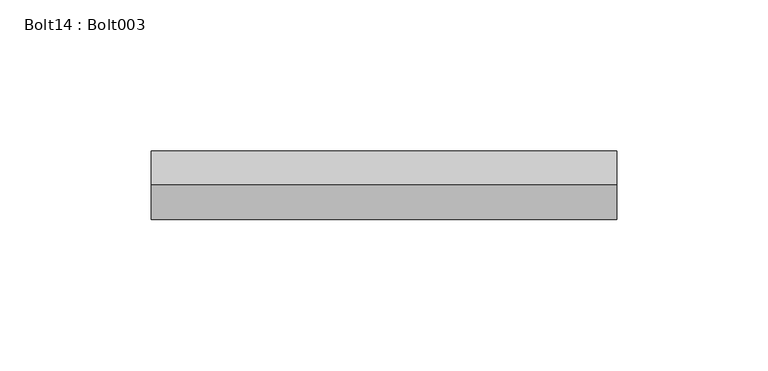
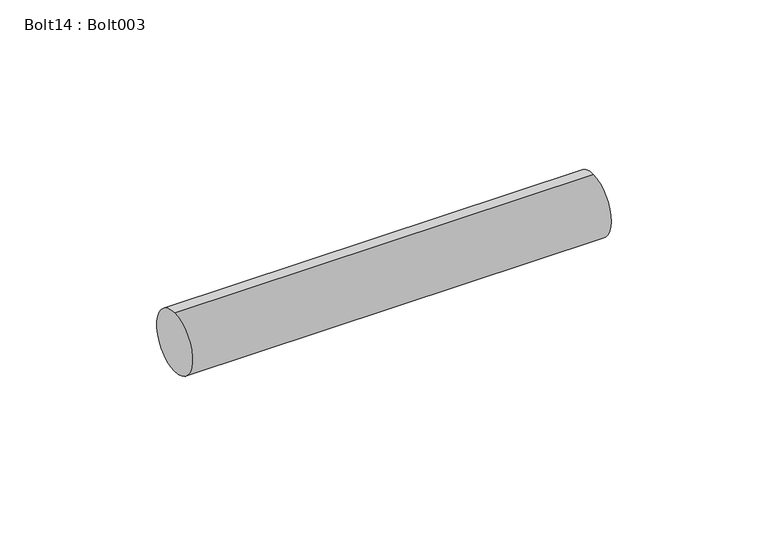
"""IFC4 building model written with IfcOpenShell, lengths in millimetres: proxy geometry, Bolt14 : Bolt003."""

import ifcopenshell
import ifcopenshell.guid

model = None  # the IFC model being written
_history = None  # IfcOwnerHistory: only IFC2X3 demands one
_inside = {}  # id of a spatial element -> (the spatial element, [elements in it])
_under = {}  # id of a project, library or spatial element -> (it, [spatial elements below it])
_declared = {}  # id of a project -> (the project, [libraries it declares])
_typed = {}  # id of a type object -> (the type object, [elements of that type])
_made_of = {}  # id of a material, layer set ... -> (it, [elements and type objects made of it])


def new_model(schema):
    """Start an empty IFC model of exactly this schema.

    Asked for "IFC4X3", IfcOpenShell would pick the latest addendum, in which some entities
    have other attributes; the version numbers below select the first issue.
    IFC2X3 requires an IfcOwnerHistory on every rooted entity: one is made here for all.
    """
    global model, _history
    if schema == "IFC4X3":
        model = ifcopenshell.file(schema_version=(4, 3, 0, 0))
    else:
        model = ifcopenshell.file(schema=schema)
    _inside.clear()
    _under.clear()
    _declared.clear()
    _typed.clear()
    _made_of.clear()
    _history = None
    if model.schema == "IFC2X3":
        org = make("IfcOrganization", Name="unknown")
        user = make(
            "IfcPersonAndOrganization",
            ThePerson=make("IfcPerson", FamilyName="unknown"),
            TheOrganization=org,
        )
        app = make(
            "IfcApplication",
            ApplicationDeveloper=org,
            Version="unknown",
            ApplicationFullName="unknown",
            ApplicationIdentifier="unknown",
        )
        _history = make(
            "IfcOwnerHistory",
            OwningUser=user,
            OwningApplication=app,
            ChangeAction="ADDED",
            CreationDate=0,
        )
    return model


def make(cls, **values):
    """One entity of the class cls with the attributes given. An attribute that is None is left unset."""
    return model.create_entity(
        cls, **{name: value for name, value in values.items() if value is not None}
    )


def rooted(cls, **values):
    """An entity with a GlobalId (a new one), such as an element, a storey or a relation."""
    return make(cls, GlobalId=ifcopenshell.guid.new(), OwnerHistory=_history, **values)


def si_unit(unit_type, name, prefix=None):
    """IfcSIUnit, for example si_unit("LENGTHUNIT", "METRE", prefix="MILLI")."""
    return make("IfcSIUnit", UnitType=unit_type, Prefix=prefix, Name=name)


def assignment(units):
    """IfcUnitAssignment: the units of a project."""
    return None if units is None else make("IfcUnitAssignment", Units=units)


def point(xyz):
    """IfcCartesianPoint."""
    return None if xyz is None else make("IfcCartesianPoint", Coordinates=xyz)


def direction(xyz):
    """IfcDirection."""
    return None if xyz is None else make("IfcDirection", DirectionRatios=xyz)


def frame(location, z_axis=None, x_axis=None):
    """IfcAxis2Placement3D, a coordinate frame: its origin and axes. An axis left out is left unset."""
    return make(
        "IfcAxis2Placement3D",
        Location=point(location),
        Axis=direction(z_axis),
        RefDirection=direction(x_axis),
    )


def frame_2d(location, x_axis=None):
    """IfcAxis2Placement2D, a coordinate frame in the plane: its origin and x axis."""
    return make(
        "IfcAxis2Placement2D", Location=point(location), RefDirection=direction(x_axis)
    )


def origin():
    """The frame at (0, 0, 0) with its axes left unset."""
    return frame((0.0, 0.0, 0.0))


def place(relative_to, where):
    """IfcLocalPlacement: puts the frame where relative to a parent placement (None: the world)."""
    return make(
        "IfcLocalPlacement", PlacementRelTo=relative_to, RelativePlacement=where
    )


def context(
    kind, dimensions, precision=None, world=None, true_north=None, identifier=None
):
    """IfcGeometricRepresentationContext, for example the 3D "Model" context."""
    return make(
        "IfcGeometricRepresentationContext",
        ContextIdentifier=identifier,
        ContextType=kind,
        CoordinateSpaceDimension=dimensions,
        Precision=precision,
        WorldCoordinateSystem=world,
        TrueNorth=true_north,
    )


def project(units=None, contexts=None):
    """IfcProject with its units and contexts."""
    return rooted(
        "IfcProject",
        Name="project",
        RepresentationContexts=contexts,
        UnitsInContext=assignment(units),
    )


def spatial(cls, under=None, at=None, **own):
    """A site, building, storey or space (cls), placed at a placement, below another one or the project."""
    s = rooted(cls, ObjectPlacement=at, **own)
    if under is not None:
        _under.setdefault(under.id(), (under, []))[1].append(s)
    return s


def circle_curve(where, radius):
    """IfcCircle in the frame where."""
    return make("IfcCircle", Position=where, Radius=radius)


def trimmed(basis, trim1, trim2, sense, master):
    """IfcTrimmedCurve: the piece of a basis curve between two trims."""
    return make(
        "IfcTrimmedCurve",
        BasisCurve=basis,
        Trim1=trim1,
        Trim2=trim2,
        SenseAgreement=sense,
        MasterRepresentation=master,
    )


def segment(curve, same_sense, transition):
    """IfcCompositeCurveSegment."""
    return make(
        "IfcCompositeCurveSegment",
        Transition=transition,
        SameSense=same_sense,
        ParentCurve=curve,
    )


def composite_curve(segments, self_intersect=None):
    """IfcCompositeCurve: segments joined end to end."""
    return make("IfcCompositeCurve", Segments=segments, SelfIntersect=self_intersect)


def outline(outer, holes=None, kind="AREA"):
    """IfcArbitraryClosedProfileDef: a profile drawn as a closed curve; with holes, ...WithVoids."""
    if holes is None:
        return make("IfcArbitraryClosedProfileDef", ProfileType=kind, OuterCurve=outer)
    return make(
        "IfcArbitraryProfileDefWithVoids",
        ProfileType=kind,
        OuterCurve=outer,
        InnerCurves=holes,
    )


def extrude(swept, where, along, depth):
    """IfcExtrudedAreaSolid: the profile swept, set in the frame where, extruded along a direction by depth."""
    return make(
        "IfcExtrudedAreaSolid",
        SweptArea=swept,
        Position=where,
        ExtrudedDirection=direction(along),
        Depth=depth,
    )


def shape(context_of_items, identifier, shape_type, items):
    """IfcShapeRepresentation: the items that make up one representation, for example the "Body"."""
    return make(
        "IfcShapeRepresentation",
        ContextOfItems=context_of_items,
        RepresentationIdentifier=identifier,
        RepresentationType=shape_type,
        Items=items,
    )


def source(mapping_origin, context_of_items, identifier, shape_type, items):
    """IfcRepresentationMap: a shape defined once, which mapped items show again and again."""
    return make(
        "IfcRepresentationMap",
        MappingOrigin=mapping_origin,
        MappedRepresentation=shape(context_of_items, identifier, shape_type, items),
    )


def transform(
    local_origin,
    x_axis=None,
    y_axis=None,
    z_axis=None,
    scale=None,
    scale2=None,
    scale3=None,
    uniform=True,
):
    """IfcCartesianTransformationOperator3D, or its non-uniform kind. x_axis, y_axis, z_axis: its Axis1, 2, 3."""
    if uniform:
        return make(
            "IfcCartesianTransformationOperator3D",
            Axis1=direction(x_axis),
            Axis2=direction(y_axis),
            LocalOrigin=point(local_origin),
            Scale=scale,
            Axis3=direction(z_axis),
        )
    return make(
        "IfcCartesianTransformationOperator3DnonUniform",
        Axis1=direction(x_axis),
        Axis2=direction(y_axis),
        LocalOrigin=point(local_origin),
        Scale=scale,
        Axis3=direction(z_axis),
        Scale2=scale2,
        Scale3=scale3,
    )


def mapped(mapping_source, mapping_target):
    """IfcMappedItem: shows the shape of a source again, moved by a transform."""
    return make(
        "IfcMappedItem", MappingSource=mapping_source, MappingTarget=mapping_target
    )


def made_of(thing, what):
    """Note that an element or type object is made of a material, layer set ...; save() writes the relation."""
    if what is not None:
        _made_of.setdefault(what.id(), (what, []))[1].append(thing)
    return thing


def element(
    cls,
    number,
    at=None,
    inside=None,
    cuts=None,
    type_object=None,
    material=None,
    context=None,
    identifier="Body",
    shape_type=None,
    held_by="IfcProductDefinitionShape",
    body=None,
    shapes=None,
    **own,
):
    """One element of the class cls, such as IfcWall. Its Tag is "e" and its number.

    at: its placement. inside: the storey or other place that contains it. cuts: it is an
    opening in that element (IfcRelVoidsElement). A single representation is given by context,
    identifier, shape_type and body (its items); several are given by shapes. held_by: the class
    of the entity that holds the representations. save() writes the other relations.
    """
    e = rooted(cls, Tag="e%d" % number, ObjectPlacement=at, **own)
    if body is not None:
        shapes = [shape(context, identifier, shape_type, body)]
    if shapes is not None:
        e.Representation = make(held_by, Representations=shapes)
    if inside is not None:
        _inside.setdefault(inside.id(), (inside, []))[1].append(e)
    if cuts is not None:
        rooted(
            "IfcRelVoidsElement", RelatingBuildingElement=cuts, RelatedOpeningElement=e
        )
    if type_object is not None:
        _typed.setdefault(type_object.id(), (type_object, []))[1].append(e)
    return made_of(e, material)


def aggregate(whole, parts):
    """IfcRelAggregates: a whole, such as a stair, and the parts it consists of."""
    return rooted("IfcRelAggregates", RelatingObject=whole, RelatedObjects=parts)


def save(model, path):
    """Write the relations noted so far, then the file.

    IfcRelAggregates (storeys below a building ...), IfcRelContainedInSpatialStructure (elements
    in a storey), IfcRelDefinesByType, IfcRelAssociatesMaterial and IfcRelDeclares: one each for
    every whole, place, type object, material and project.
    """
    for whole, parts in _under.values():
        aggregate(whole, parts)
    for where, things in _inside.values():
        rooted(
            "IfcRelContainedInSpatialStructure",
            RelatedElements=things,
            RelatingStructure=where,
        )
    for kind, things in _typed.values():
        rooted("IfcRelDefinesByType", RelatedObjects=things, RelatingType=kind)
    for what, things in _made_of.values():
        rooted("IfcRelAssociatesMaterial", RelatedObjects=things, RelatingMaterial=what)
    for by, libraries in _declared.values():
        rooted("IfcRelDeclares", RelatingContext=by, RelatedDefinitions=libraries)
    model.write(path)


def bolt14_bolt003_cd8d5e77(model_context):
    return source(origin(), model_context, "Body", "SweptSolid", [
        extrude(outline(composite_curve([segment(trimmed(circle_curve(frame_2d((1896.5882072, 40070.0545241)), 11.4045168), [point((1896.5882072, 40058.6500073))], [point((1896.5882072, 40081.4590409))], False, "CARTESIAN"), True, "CONTINUOUS"), segment(trimmed(circle_curve(frame_2d((1896.5882072, 40070.0545241)), 11.4045168), [point((1896.5882072, 40081.4590409))], [point((1896.5882072, 40058.6500073))], False, "CARTESIAN"), True, "CONTINUOUS")], self_intersect=False)), frame((10287.3140827, 0.0, 0.0), z_axis=(1.0, 0.0, 0.0), x_axis=(0.0, 1.0, 0.0)), (0.0, 0.0, 1.0), 154.0602393),
    ])


if __name__ == "__main__":
    model = new_model("IFC4")
    model_context = context("Model", 3, world=origin())
    ifc_project = project(units=[si_unit("LENGTHUNIT", "METRE", prefix="MILLI")], contexts=[model_context])
    site = spatial("IfcSite", under=ifc_project)
    building = spatial("IfcBuilding", under=site)
    placement = place(None, origin())
    bolt14_bolt003_shape = bolt14_bolt003_cd8d5e77(model_context)
    element("IfcBuildingElementProxy", 1, Name="Bolt14 : Bolt003", ObjectType="Bolt14 : Bolt003", at=placement, inside=building, context=model_context, shape_type="MappedRepresentation", body=[
        mapped(bolt14_bolt003_shape, transform((0.0, 0.0, 0.0), x_axis=(1.0, 0.0, 0.0), y_axis=(0.0, 1.0, 0.0), z_axis=(0.0, 0.0, 1.0))),
    ])
    save(model, "model.ifc")

# Revit data of these elements
# Type "Bolt14 : Bolt003"
#   NameOverride = "Bolt003"
# Element 1 (IfcBuildingElementProxy, "Bolt14 : Bolt003")
#   Materials on its faces: "TUBE STEEL STRINGER WELDED TO ANCHORED STEEL PLATE - SEE STRUCT DWGS"
# Materials
#   "TUBE STEEL STRINGER WELDED TO ANCHORED STEEL PLATE - SEE STRUCT DWGS": class "Unassigned", colour RGB 128 128 128, transparency 0, Cost = 0
